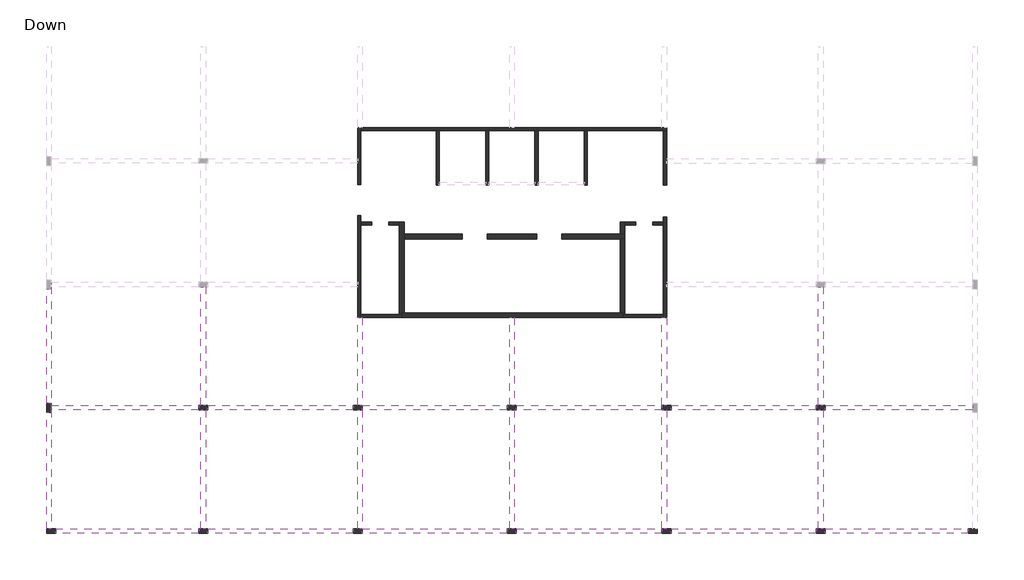
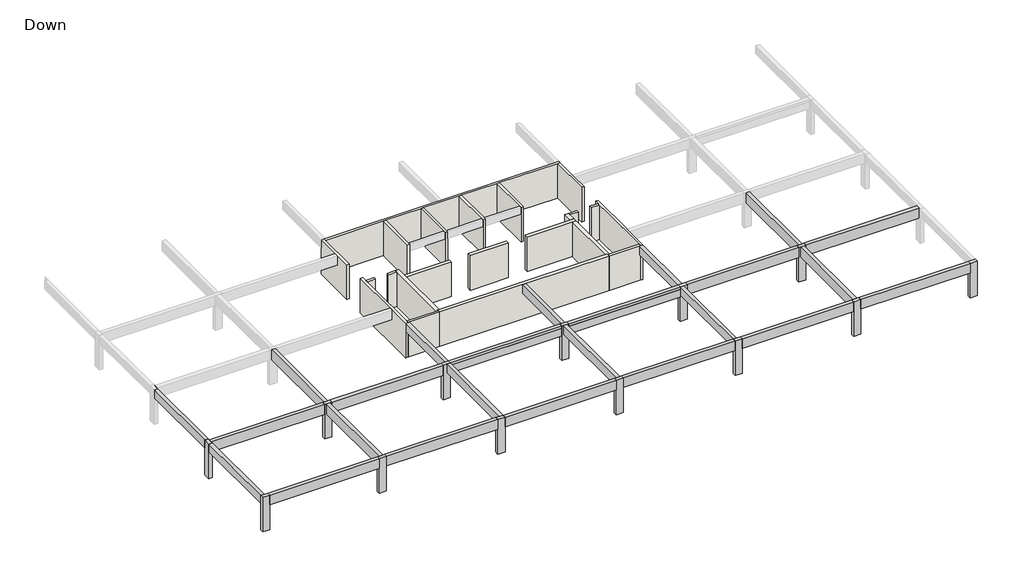
# One storey, part 1 of 2: 24 beams, 22 walls, 13 columns.
"""IFC4 building model written with IfcOpenShell, lengths in millimetres."""

import ifcopenshell
import ifcopenshell.guid

model = None  # the IFC model being written
_history = None  # IfcOwnerHistory: only IFC2X3 demands one
_inside = {}  # id of a spatial element -> (the spatial element, [elements in it])
_under = {}  # id of a project, library or spatial element -> (it, [spatial elements below it])
_declared = {}  # id of a project -> (the project, [libraries it declares])
_typed = {}  # id of a type object -> (the type object, [elements of that type])
_made_of = {}  # id of a material, layer set ... -> (it, [elements and type objects made of it])


def new_model(schema):
    """Start an empty IFC model of exactly this schema.

    Asked for "IFC4X3", IfcOpenShell would pick the latest addendum, in which some entities
    have other attributes; the version numbers below select the first issue.
    IFC2X3 requires an IfcOwnerHistory on every rooted entity: one is made here for all.
    """
    global model, _history
    if schema == "IFC4X3":
        model = ifcopenshell.file(schema_version=(4, 3, 0, 0))
    else:
        model = ifcopenshell.file(schema=schema)
    _inside.clear()
    _under.clear()
    _declared.clear()
    _typed.clear()
    _made_of.clear()
    _history = None
    if model.schema == "IFC2X3":
        org = make("IfcOrganization", Name="unknown")
        user = make(
            "IfcPersonAndOrganization",
            ThePerson=make("IfcPerson", FamilyName="unknown"),
            TheOrganization=org,
        )
        app = make(
            "IfcApplication",
            ApplicationDeveloper=org,
            Version="unknown",
            ApplicationFullName="unknown",
            ApplicationIdentifier="unknown",
        )
        _history = make(
            "IfcOwnerHistory",
            OwningUser=user,
            OwningApplication=app,
            ChangeAction="ADDED",
            CreationDate=0,
        )
    return model


def make(cls, **values):
    """One entity of the class cls with the attributes given. An attribute that is None is left unset."""
    return model.create_entity(
        cls, **{name: value for name, value in values.items() if value is not None}
    )


def rooted(cls, **values):
    """An entity with a GlobalId (a new one), such as an element, a storey or a relation."""
    return make(cls, GlobalId=ifcopenshell.guid.new(), OwnerHistory=_history, **values)


def si_unit(unit_type, name, prefix=None):
    """IfcSIUnit, for example si_unit("LENGTHUNIT", "METRE", prefix="MILLI")."""
    return make("IfcSIUnit", UnitType=unit_type, Prefix=prefix, Name=name)


def assignment(units):
    """IfcUnitAssignment: the units of a project."""
    return None if units is None else make("IfcUnitAssignment", Units=units)


def point(xyz):
    """IfcCartesianPoint."""
    return None if xyz is None else make("IfcCartesianPoint", Coordinates=xyz)


def direction(xyz):
    """IfcDirection."""
    return None if xyz is None else make("IfcDirection", DirectionRatios=xyz)


def frame(location, z_axis=None, x_axis=None):
    """IfcAxis2Placement3D, a coordinate frame: its origin and axes. An axis left out is left unset."""
    return make(
        "IfcAxis2Placement3D",
        Location=point(location),
        Axis=direction(z_axis),
        RefDirection=direction(x_axis),
    )


def origin():
    """The frame at (0, 0, 0) with its axes left unset."""
    return frame((0.0, 0.0, 0.0))


def origin_with_axes():
    """The frame at (0, 0, 0) with the z axis (0, 0, 1) and the x axis (1, 0, 0) written out."""
    return frame((0.0, 0.0, 0.0), z_axis=(0.0, 0.0, 1.0), x_axis=(1.0, 0.0, 0.0))


def place(relative_to, where):
    """IfcLocalPlacement: puts the frame where relative to a parent placement (None: the world)."""
    return make(
        "IfcLocalPlacement", PlacementRelTo=relative_to, RelativePlacement=where
    )


def context(
    kind, dimensions, precision=None, world=None, true_north=None, identifier=None
):
    """IfcGeometricRepresentationContext, for example the 3D "Model" context."""
    return make(
        "IfcGeometricRepresentationContext",
        ContextIdentifier=identifier,
        ContextType=kind,
        CoordinateSpaceDimension=dimensions,
        Precision=precision,
        WorldCoordinateSystem=world,
        TrueNorth=true_north,
    )


def project(units=None, contexts=None):
    """IfcProject with its units and contexts."""
    return rooted(
        "IfcProject",
        Name="project",
        RepresentationContexts=contexts,
        UnitsInContext=assignment(units),
    )


def spatial(cls, under=None, at=None, **own):
    """A site, building, storey or space (cls), placed at a placement, below another one or the project."""
    s = rooted(cls, ObjectPlacement=at, **own)
    if under is not None:
        _under.setdefault(under.id(), (under, []))[1].append(s)
    return s


def polyline(points):
    """IfcPolyline through the points."""
    return make("IfcPolyline", Points=[point(p) for p in points])


def outline(outer, holes=None, kind="AREA"):
    """IfcArbitraryClosedProfileDef: a profile drawn as a closed curve; with holes, ...WithVoids."""
    if holes is None:
        return make("IfcArbitraryClosedProfileDef", ProfileType=kind, OuterCurve=outer)
    return make(
        "IfcArbitraryProfileDefWithVoids",
        ProfileType=kind,
        OuterCurve=outer,
        InnerCurves=holes,
    )


def extrude(swept, where, along, depth):
    """IfcExtrudedAreaSolid: the profile swept, set in the frame where, extruded along a direction by depth."""
    return make(
        "IfcExtrudedAreaSolid",
        SweptArea=swept,
        Position=where,
        ExtrudedDirection=direction(along),
        Depth=depth,
    )


def faces_of(points, faces, orient=None, outer=None):
    """IfcFace entities. A face is a list of loops; a loop is a list of indices into points, from 0.

    orient and outer hold one flag for each loop. By default every Orientation is true, the
    first loop of a face is its IfcFaceOuterBound and the others are IfcFaceBound.
    """
    made = []
    for i, loops in enumerate(faces):
        bounds = []
        for j, loop in enumerate(loops):
            is_outer = j == 0 if outer is None else outer[i][j]
            bounds.append(
                make(
                    "IfcFaceOuterBound" if is_outer else "IfcFaceBound",
                    Bound=make("IfcPolyLoop", Polygon=[points[k] for k in loop]),
                    Orientation=True if orient is None else orient[i][j],
                )
            )
        made.append(make("IfcFace", Bounds=bounds))
    return made


def faceted_brep(points, faces, orient=None, outer=None, voids=None):
    """IfcFacetedBrep: a solid bounded by flat faces; with voids (closed shells), ...WithVoids."""
    shared = [point(p) for p in points]
    hull = make("IfcClosedShell", CfsFaces=faces_of(shared, faces, orient, outer))
    if voids is None:
        return make("IfcFacetedBrep", Outer=hull)
    return make(
        "IfcFacetedBrepWithVoids",
        Outer=hull,
        Voids=[
            make(cls, CfsFaces=faces_of(shared, fs, o, b)) for cls, fs, o, b in voids
        ],
    )


def shape(context_of_items, identifier, shape_type, items):
    """IfcShapeRepresentation: the items that make up one representation, for example the "Body"."""
    return make(
        "IfcShapeRepresentation",
        ContextOfItems=context_of_items,
        RepresentationIdentifier=identifier,
        RepresentationType=shape_type,
        Items=items,
    )


def made_of(thing, what):
    """Note that an element or type object is made of a material, layer set ...; save() writes the relation."""
    if what is not None:
        _made_of.setdefault(what.id(), (what, []))[1].append(thing)
    return thing


def element(
    cls,
    number,
    at=None,
    inside=None,
    cuts=None,
    type_object=None,
    material=None,
    context=None,
    identifier="Body",
    shape_type=None,
    held_by="IfcProductDefinitionShape",
    body=None,
    shapes=None,
    **own,
):
    """One element of the class cls, such as IfcWall. Its Tag is "e" and its number.

    at: its placement. inside: the storey or other place that contains it. cuts: it is an
    opening in that element (IfcRelVoidsElement). A single representation is given by context,
    identifier, shape_type and body (its items); several are given by shapes. held_by: the class
    of the entity that holds the representations. save() writes the other relations.
    """
    e = rooted(cls, Tag="e%d" % number, ObjectPlacement=at, **own)
    if body is not None:
        shapes = [shape(context, identifier, shape_type, body)]
    if shapes is not None:
        e.Representation = make(held_by, Representations=shapes)
    if inside is not None:
        _inside.setdefault(inside.id(), (inside, []))[1].append(e)
    if cuts is not None:
        rooted(
            "IfcRelVoidsElement", RelatingBuildingElement=cuts, RelatedOpeningElement=e
        )
    if type_object is not None:
        _typed.setdefault(type_object.id(), (type_object, []))[1].append(e)
    return made_of(e, material)


def aggregate(whole, parts):
    """IfcRelAggregates: a whole, such as a stair, and the parts it consists of."""
    return rooted("IfcRelAggregates", RelatingObject=whole, RelatedObjects=parts)


def save(model, path):
    """Write the relations noted so far, then the file.

    IfcRelAggregates (storeys below a building ...), IfcRelContainedInSpatialStructure (elements
    in a storey), IfcRelDefinesByType, IfcRelAssociatesMaterial and IfcRelDeclares: one each for
    every whole, place, type object, material and project.
    """
    for whole, parts in _under.values():
        aggregate(whole, parts)
    for where, things in _inside.values():
        rooted(
            "IfcRelContainedInSpatialStructure",
            RelatedElements=things,
            RelatingStructure=where,
        )
    for kind, things in _typed.values():
        rooted("IfcRelDefinesByType", RelatedObjects=things, RelatingType=kind)
    for what, things in _made_of.values():
        rooted("IfcRelAssociatesMaterial", RelatedObjects=things, RelatingMaterial=what)
    for by, libraries in _declared.values():
        rooted("IfcRelDeclares", RelatingContext=by, RelatedDefinitions=libraries)
    model.write(path)


model = new_model("IFC4")

# Units and contexts
model_context = context("Model", 3, world=origin())
ifc_project = project(units=[si_unit("LENGTHUNIT", "METRE", prefix="MILLI")], contexts=[model_context])

# Site, building, storey
site = spatial("IfcSite", under=ifc_project)
building = spatial("IfcBuilding", under=site)
storey = spatial("IfcBuildingStorey", under=building, Name="Down", Elevation=0.0)

# Beams
placement = place(None, origin())
element("IfcBeam", 1, ObjectType="Concrete Rectengular Beam : 30/70", at=placement, inside=storey, context=model_context, shape_type="Brep", body=[
    faceted_brep([(-26599.1167382, -14918.7716477, 3080.0), (-26299.1167382, -14918.7716477, 3080.0), (-26299.1167382, -7220.4648963, 3080.0), (-26299.1167382, -6920.4648963, 3080.0), (-26299.591421, -6920.4648963, 3080.0), (-26299.591421, -7370.4648963, 3080.0), (-26599.1167382, -7370.4648963, 3080.0), (-26299.1167382, -14918.7716477, 2860.0), (-26299.1167382, -14918.7716477, 2380.0), (-26299.1167382, -7220.4648963, 2380.0), (-26299.1167382, -6920.4648963, 2380.0), (-26599.1167382, -14918.7716477, 2380.0), (-26599.1167382, -7370.4648963, 2380.0), (-26299.591421, -7370.4648963, 2380.0), (-26299.591421, -7220.4648963, 2380.0), (-26299.591421, -6920.4648963, 2380.0)], [[[0, 1, 2, 3, 4, 5, 6]], [[1, 7, 8, 9, 10, 3, 2]], [[8, 11, 12, 13, 14, 15, 10, 9]], [[11, 0, 6, 12]], [[1, 0, 11, 8, 7]], [[13, 5, 4, 15, 14]], [[5, 13, 12, 6]], [[3, 10, 15, 4]]]),
])
element("IfcBeam", 2, ObjectType="Concrete Rectengular Beam : 30/70", at=placement, inside=storey, context=model_context, shape_type="Brep", body=[
    faceted_brep([(-26599.1167382, -6770.4648963, 3080.0), (-26299.591421, -6770.4648963, 3080.0), (-26299.591421, -6920.4648963, 3080.0), (-26299.1167382, -6920.4648963, 3080.0), (-26299.1167382, 774.102585, 3080.0), (-26299.1167382, 1074.102585, 3080.0), (-26299.591421, 1074.102585, 3080.0), (-26299.591421, 624.102585, 3080.0), (-26599.1167382, 624.102585, 3080.0), (-26299.1167382, 1074.102585, 2380.0), (-26299.1167382, -6920.4648963, 2860.0), (-26299.1167382, -6920.4648963, 2380.0), (-26299.1167382, 774.102585, 2380.0), (-26299.591421, -6770.4648963, 2380.0), (-26599.1167382, -6770.4648963, 2380.0), (-26599.1167382, 624.102585, 2380.0), (-26299.591421, 624.102585, 2380.0), (-26299.591421, 774.102585, 2380.0), (-26299.591421, 1074.102585, 2380.0), (-26299.591421, -6920.4648963, 2380.0)], [[[0, 1, 2, 3, 4, 5, 6, 7, 8]], [[9, 5, 4, 3, 10, 11, 12]], [[13, 14, 15, 16, 17, 18, 9, 12, 11, 19]], [[14, 0, 8, 15]], [[13, 1, 0, 14]], [[1, 13, 19, 2]], [[16, 7, 6, 18, 17]], [[7, 16, 15, 8]], [[5, 9, 18, 6]], [[11, 10, 3, 2, 19]]]),
])
element("IfcBeam", 3, ObjectType="Concrete Rectengular Beam : 30/75", at=placement, inside=storey, context=model_context, shape_type="Brep", body=[
    faceted_brep([(-6147.328783, -7220.4648963, 3080.0), (-6447.328783, -7220.4648963, 3080.0), (-6447.328783, -14918.7716477, 3080.0), (-6147.328783, -14918.7716477, 3080.0), (-6147.328783, -7220.4648963, 2330.0), (-6147.328783, -14918.7716477, 2330.0), (-6447.328783, -7220.4648963, 2330.0), (-6447.328783, -14918.7716477, 2330.0), (-6447.328783, -7220.4648963, 2860.0), (-6447.328783, -14918.7716477, 2860.0)], [[[0, 1, 2, 3]], [[4, 0, 3, 5]], [[6, 4, 5, 7]], [[1, 8, 6, 7, 9, 2]], [[1, 0, 4, 6, 8]], [[3, 2, 9, 7, 5]]]),
])
element("IfcBeam", 4, ObjectType="Concrete Rectengular Beam : 30/75", at=placement, inside=storey, context=model_context, shape_type="Brep", body=[
    faceted_brep([(-6447.328783, -6920.4648963, 3080.0), (-6147.328783, -6920.4648963, 3080.0), (-6147.328783, -1210.4648963, 3080.0), (-6247.328783, -1210.4648963, 3080.0), (-6447.328783, -1210.4648963, 3080.0), (-6147.328783, -6920.4648963, 2860.0), (-6147.328783, -6920.4648963, 2330.0), (-6147.328783, -1210.4648963, 2330.0), (-6147.328783, -1210.4648963, 2860.0), (-6447.328783, -6920.4648963, 2330.0), (-6447.328783, -1210.4648963, 2330.0), (-6447.328783, -6920.4648963, 2860.0)], [[[0, 1, 2, 3, 4]], [[1, 5, 6, 7, 8, 2]], [[6, 9, 10, 7]], [[9, 11, 0, 4, 10]], [[1, 0, 11, 9, 6, 5]], [[2, 8, 7, 10, 4, 3]]]),
])
element("IfcBeam", 5, ObjectType="Concrete Rectengular Beam : 30/75", at=placement, inside=storey, context=model_context, shape_type="Brep", body=[
    faceted_brep([(3389.2018335, -6920.4648963, 3080.0), (3689.2018335, -6920.4648963, 3080.0), (3689.2018335, -1210.4648963, 3080.0), (3389.2018335, -1210.4648963, 3080.0), (3689.2018335, -6920.4648963, 2860.0), (3689.2018335, -6920.4648963, 2330.0), (3689.2018335, -1210.4648963, 2330.0), (3689.2018335, -1210.4648963, 2860.0), (3389.2018335, -6920.4648963, 2330.0), (3389.2018335, -1210.4648963, 2330.0), (3389.2018335, -6920.4648963, 2860.0), (3389.2018335, -1210.4648963, 2860.0)], [[[0, 1, 2, 3]], [[1, 4, 5, 6, 7, 2]], [[5, 8, 9, 6]], [[8, 10, 0, 3, 11, 9]], [[1, 0, 10, 8, 5, 4]], [[3, 2, 7, 6, 9, 11]]]),
])
element("IfcBeam", 6, ObjectType="Concrete Rectengular Beam : 30/75", at=placement, inside=storey, context=model_context, shape_type="Brep", body=[
    faceted_brep([(3389.2018335, -14918.7716477, 3080.0), (3689.2018335, -14918.7716477, 3080.0), (3689.2018335, -7220.4648963, 3080.0), (3389.2018335, -7220.4648963, 3080.0), (3389.2018335, -14918.7716477, 2330.0), (3389.2018335, -14918.7716477, 2860.0), (3389.2018335, -7220.4648963, 2860.0), (3389.2018335, -7220.4648963, 2330.0), (3689.2018335, -14918.7716477, 2330.0), (3689.2018335, -7220.4648963, 2330.0), (3689.2018335, -14918.7716477, 2860.0), (3689.2018335, -7220.4648963, 2860.0)], [[[0, 1, 2, 3]], [[4, 5, 0, 3, 6, 7]], [[8, 4, 7, 9]], [[1, 10, 8, 9, 11, 2]], [[1, 0, 5, 4, 8, 10]], [[3, 2, 11, 9, 7, 6]]]),
])
element("IfcBeam", 7, ObjectType="Concrete Rectengular Beam : 30/75", at=placement, inside=storey, context=model_context, shape_type="SweptSolid", body=[
    extrude(outline(polyline([(2330.0, 13257.9839294), (2330.0, 13557.9839294), (2860.0, 13557.9839294), (2860.0, 13525.73245), (3080.0, 13525.73245), (3080.0, 13257.9839294), (2330.0, 13257.9839294)])), frame((0.0, -14918.7716477, 0.0), z_axis=(0.0, 1.0, 0.0), x_axis=(0.0, 0.0, 1.0)), (0.0, 0.0, 1.0), 7698.3067514),
])
element("IfcBeam", 8, ObjectType="Concrete Rectengular Beam : 30/75", at=placement, inside=storey, context=model_context, shape_type="Brep", body=[
    faceted_brep([(13257.9839294, -6920.4648963, 3080.0), (13557.9839294, -6920.4648963, 3080.0), (13557.9839294, -1210.4648963, 3080.0), (13357.9839294, -1210.4648963, 3080.0), (13257.9839294, -1210.4648963, 3080.0), (13557.9839294, -6920.4648963, 2860.0), (13557.9839294, -6920.4648963, 2330.0), (13557.9839294, -1210.4648963, 2330.0), (13257.9839294, -6920.4648963, 2330.0), (13257.9839294, -1210.4648963, 2330.0), (13257.9839294, -6920.4648963, 2860.0), (13257.9839294, -1210.4648963, 2860.0)], [[[0, 1, 2, 3, 4]], [[1, 5, 6, 7, 2]], [[6, 8, 9, 7]], [[8, 10, 0, 4, 11, 9]], [[1, 0, 10, 8, 6, 5]], [[2, 7, 9, 11, 4, 3]]]),
])
element("IfcBeam", 9, ObjectType="Concrete Rectengular Beam : 30/85", at=placement, inside=storey, context=model_context, shape_type="SweptSolid", body=[
    extrude(outline(polyline([(33098.6447783, -14918.7716477), (33098.6447783, -15218.7716477), (23850.3644839, -15218.7716477), (23850.3644839, -14918.7716477), (33098.6447783, -14918.7716477)])), frame((0.0, 0.0, 2230.0), z_axis=(0.0, 0.0, 1.0), x_axis=(1.0, 0.0, 0.0)), (0.0, 0.0, 1.0), 850.0),
])
element("IfcBeam", 10, ObjectType="Concrete Rectengular Beam : 30/85", at=placement, inside=storey, context=model_context, shape_type="SweptSolid", body=[
    extrude(outline(polyline([(23250.3644839, -14918.7716477), (23250.3644839, -15218.7716477), (13857.9839294, -15218.7716477), (13857.9839294, -14918.7716477), (23250.3644839, -14918.7716477)])), frame((0.0, 0.0, 2230.0), z_axis=(0.0, 0.0, 1.0), x_axis=(1.0, 0.0, 0.0)), (0.0, 0.0, 1.0), 850.0),
])
element("IfcBeam", 11, ObjectType="Concrete Rectengular Beam : 30/85", at=placement, inside=storey, context=model_context, shape_type="SweptSolid", body=[
    extrude(outline(polyline([(-14918.7716477, 2230.0), (-15218.7716477, 2230.0), (-15218.7716477, 3080.0), (-14922.522162, 3080.0), (-14922.522162, 2860.0), (-14918.7716477, 2860.0), (-14918.7716477, 2230.0)])), frame((3839.2018335, 0.0, 0.0), z_axis=(1.0, 0.0, 0.0), x_axis=(0.0, 1.0, 0.0)), (0.0, 0.0, 1.0), 9418.7820959),
])
element("IfcBeam", 12, ObjectType="Concrete Rectengular Beam : 30/85", at=placement, inside=storey, context=model_context, shape_type="SweptSolid", body=[
    extrude(outline(polyline([(-14918.7716477, 2230.0), (-15218.7716477, 2230.0), (-15218.7716477, 3080.0), (-14922.522162, 3080.0), (-14922.522162, 2860.0), (-14918.7716477, 2860.0), (-14918.7716477, 2230.0)])), frame((-6147.328783, 0.0, 0.0), z_axis=(1.0, 0.0, 0.0), x_axis=(0.0, 1.0, 0.0)), (0.0, 0.0, 1.0), 9386.5306165),
])
element("IfcBeam", 13, ObjectType="Concrete Rectengular Beam : 30/85", at=placement, inside=storey, context=model_context, shape_type="SweptSolid", body=[
    extrude(outline(polyline([(-16150.7819865, -15218.7716477), (-16150.7819865, -14918.7716477), (-6747.328783, -14918.7716477), (-6747.328783, -15218.7716477), (-16150.7819865, -15218.7716477)])), frame((0.0, 0.0, 2230.0), z_axis=(0.0, 0.0, 1.0), x_axis=(1.0, 0.0, 0.0)), (0.0, 0.0, 1.0), 850.0),
])
element("IfcBeam", 14, ObjectType="Concrete Rectengular Beam : 30/85", at=placement, inside=storey, context=model_context, shape_type="SweptSolid", body=[
    extrude(outline(polyline([(-25999.1167382, -15218.7716477), (-25999.1167382, -14918.7716477), (-16750.7819865, -14918.7716477), (-16750.7819865, -15218.7716477), (-25999.1167382, -15218.7716477)])), frame((0.0, 0.0, 2230.0), z_axis=(0.0, 0.0, 1.0), x_axis=(1.0, 0.0, 0.0)), (0.0, 0.0, 1.0), 850.0),
])
element("IfcBeam", 15, ObjectType="Concrete Rectengular Beam : 30/90", at=placement, inside=storey, context=model_context, shape_type="Brep", body=[
    faceted_brep([(-16750.7819865, -7220.4648963, 3080.0), (-16750.7819865, -6920.4648963, 3080.0), (-26299.1167382, -6920.4648963, 3080.0), (-26299.1167382, -7220.4648963, 3080.0), (-16750.7819865, -7220.4648963, 2180.0), (-26299.1167382, -7220.4648963, 2860.0), (-26299.1167382, -7220.4648963, 2380.0), (-26299.591421, -7220.4648963, 2380.0), (-26299.591421, -7220.4648963, 2180.0), (-16750.7819865, -6920.4648963, 2180.0), (-26299.591421, -6920.4648963, 2180.0), (-26299.591421, -6920.4648963, 2380.0), (-26299.1167382, -6920.4648963, 2380.0), (-26299.1167382, -6920.4648963, 2860.0)], [[[0, 1, 2, 3]], [[4, 0, 3, 5, 6, 7, 8]], [[9, 4, 8, 10]], [[1, 9, 10, 11, 12, 13, 2]], [[1, 0, 4, 9]], [[10, 8, 7, 11]], [[12, 6, 5, 3, 2, 13]], [[6, 12, 11, 7]]]),
])
element("IfcBeam", 16, ObjectType="Concrete Rectengular Beam : 30/90", at=placement, inside=storey, context=model_context, shape_type="SweptSolid", body=[
    extrude(outline(polyline([(-16150.7819865, -7220.4648963), (-16150.7819865, -6920.4648963), (-6747.328783, -6920.4648963), (-6747.328783, -7220.4648963), (-16150.7819865, -7220.4648963)])), frame((0.0, 0.0, 2180.0), z_axis=(0.0, 0.0, 1.0), x_axis=(1.0, 0.0, 0.0)), (0.0, 0.0, 1.0), 900.0),
])
element("IfcBeam", 17, ObjectType="Concrete Rectengular Beam : 30/90", at=placement, inside=storey, context=model_context, shape_type="Brep", body=[
    faceted_brep([(3239.2018335, -6920.4648963, 3080.0), (-6147.328783, -6920.4648963, 3080.0), (-6147.328783, -7220.13739, 3080.0), (3239.2018335, -7220.13739, 3080.0), (-6147.328783, -7220.4648963, 2180.0), (3239.2018335, -7220.4648963, 2180.0), (3239.2018335, -7220.4648963, 2860.0), (-6147.328783, -7220.4648963, 2860.0), (3239.2018335, -6920.4648963, 2180.0), (-6147.328783, -6920.4648963, 2180.0), (-6147.328783, -6920.4648963, 2860.0), (3239.2018335, -7220.13739, 2860.0), (-6147.328783, -7220.13739, 2860.0)], [[[0, 1, 2, 3]], [[4, 5, 6, 7]], [[8, 5, 4, 9]], [[0, 8, 9, 10, 1]], [[5, 8, 0, 3, 11, 6]], [[9, 4, 7, 12, 2, 1, 10]], [[11, 12, 7, 6]], [[12, 11, 3, 2]]]),
])
element("IfcBeam", 18, ObjectType="Concrete Rectengular Beam : 30/90", at=placement, inside=storey, context=model_context, shape_type="Brep", body=[
    faceted_brep([(13257.9839294, -6920.4648963, 3080.0), (3839.2018335, -6920.4648963, 3080.0), (3839.2018335, -7220.13739, 3080.0), (13257.9839294, -7220.13739, 3080.0), (3839.2018335, -7220.4648963, 2180.0), (13257.9839294, -7220.4648963, 2180.0), (13257.9839294, -7220.4648963, 2860.0), (3839.2018335, -7220.4648963, 2860.0), (3839.2018335, -6920.4648963, 2180.0), (13257.9839294, -6920.4648963, 2180.0), (13257.9839294, -6920.4648963, 2860.0), (3839.2018335, -7220.13739, 2860.0), (13257.9839294, -7220.13739, 2860.0)], [[[0, 1, 2, 3]], [[4, 5, 6, 7]], [[4, 8, 9, 5]], [[8, 1, 0, 10, 9]], [[8, 4, 7, 11, 2, 1]], [[5, 9, 10, 0, 3, 12, 6]], [[12, 11, 7, 6]], [[11, 12, 3, 2]]]),
])
element("IfcBeam", 19, ObjectType="Concrete Rectengular Beam : 30/90", at=placement, inside=storey, context=model_context, shape_type="SweptSolid", body=[
    extrude(outline(polyline([(23250.3644839, -6920.4648963), (23250.3644839, -7220.4648963), (13857.9839294, -7220.4648963), (13857.9839294, -6920.4648963), (23250.3644839, -6920.4648963)])), frame((0.0, 0.0, 2180.0), z_axis=(0.0, 0.0, 1.0), x_axis=(1.0, 0.0, 0.0)), (0.0, 0.0, 1.0), 900.0),
])
element("IfcBeam", 20, ObjectType="Concrete Rectengular Beam : 30/90", at=placement, inside=storey, context=model_context, shape_type="Brep", body=[
    faceted_brep([(33398.6447783, -7220.4648963, 3080.0), (33398.6447783, -6920.4648963, 3080.0), (23850.3644839, -6920.4648963, 3080.0), (23850.3644839, -7220.4648963, 3080.0), (33398.6447783, -7220.4648963, 2180.0), (33398.6447783, -7220.4648963, 2860.0), (23850.3644839, -7220.4648963, 2180.0), (33398.6447783, -6920.4648963, 2180.0), (23850.3644839, -6920.4648963, 2180.0), (33398.6447783, -6920.4648963, 2860.0)], [[[0, 1, 2, 3]], [[4, 5, 0, 3, 6]], [[7, 4, 6, 8]], [[1, 9, 7, 8, 2]], [[1, 0, 5, 4, 7, 9]], [[3, 2, 8, 6]]]),
])
element("IfcBeam", 21, ObjectType="Concrete Rectengular Beam : 30/90", at=placement, inside=storey, context=model_context, shape_type="Brep", body=[
    faceted_brep([(-16600.7819865, -6920.4648963, 3080.0), (-16300.7819865, -6920.4648963, 3080.0), (-16300.7819865, 774.102585, 3080.0), (-16600.7819865, 774.102585, 3080.0), (-16600.7819865, -6920.4648963, 2180.0), (-16600.7819865, -6920.4648963, 2860.0), (-16600.7819865, 774.102585, 2860.0), (-16600.7819865, 774.102585, 2180.0), (-16300.7819865, -6920.4648963, 2180.0), (-16300.7819865, 774.102585, 2180.0), (-16300.7819865, -6920.4648963, 2860.0), (-16300.7819865, 774.102585, 2860.0)], [[[0, 1, 2, 3]], [[4, 5, 0, 3, 6, 7]], [[8, 4, 7, 9]], [[1, 10, 8, 9, 11, 2]], [[0, 5, 4, 8, 10, 1]], [[2, 11, 9, 7, 6, 3]]]),
])
element("IfcBeam", 22, ObjectType="Concrete Rectengular Beam : 30/90", at=placement, inside=storey, context=model_context, shape_type="Brep", body=[
    faceted_brep([(-16300.7819865, -7220.4648963, 3080.0), (-16600.7819865, -7220.4648963, 3080.0), (-16600.7819865, -14918.7716477, 3080.0), (-16300.7819865, -14918.7716477, 3080.0), (-16600.7819865, -7220.4648963, 2860.0), (-16600.7819865, -7220.4648963, 2180.0), (-16600.7819865, -14918.7716477, 2180.0), (-16600.7819865, -14918.7716477, 2860.0), (-16300.7819865, -7220.4648963, 2180.0), (-16300.7819865, -14918.7716477, 2180.0), (-16300.7819865, -7220.4648963, 2860.0), (-16300.7819865, -14918.7716477, 2860.0)], [[[0, 1, 2, 3]], [[1, 4, 5, 6, 7, 2]], [[5, 8, 9, 6]], [[8, 10, 0, 3, 11, 9]], [[5, 4, 1, 0, 10, 8]], [[3, 2, 7, 6, 9, 11]]]),
])
element("IfcBeam", 23, ObjectType="Concrete Rectengular Beam : 30/90", at=placement, inside=storey, context=model_context, shape_type="Brep", body=[
    faceted_brep([(23400.3644839, -6920.4648963, 3080.0), (23700.3644839, -6920.4648963, 3080.0), (23700.3644839, 774.102585, 3080.0), (23400.3644839, 774.102585, 3080.0), (23400.3644839, -6920.4648963, 2180.0), (23400.3644839, -6920.4648963, 2860.0), (23400.3644839, 774.102585, 2860.0), (23400.3644839, 774.102585, 2180.0), (23700.3644839, -6920.4648963, 2180.0), (23700.3644839, 774.102585, 2180.0), (23700.3644839, -6920.4648963, 2860.0), (23700.3644839, 774.102585, 2860.0)], [[[0, 1, 2, 3]], [[4, 5, 0, 3, 6, 7]], [[8, 4, 7, 9]], [[1, 10, 8, 9, 11, 2]], [[0, 5, 4, 8, 10, 1]], [[9, 7, 6, 3, 2, 11]]]),
])
element("IfcBeam", 24, ObjectType="Concrete Rectengular Beam : 30/90", at=placement, inside=storey, context=model_context, shape_type="Brep", body=[
    faceted_brep([(23700.3644839, -7220.4648963, 3080.0), (23400.3644839, -7220.4648963, 3080.0), (23400.3644839, -14918.7716477, 3080.0), (23700.3644839, -14918.7716477, 3080.0), (23400.3644839, -7220.4648963, 2860.0), (23400.3644839, -7220.4648963, 2180.0), (23400.3644839, -14918.7716477, 2180.0), (23400.3644839, -14918.7716477, 2860.0), (23700.3644839, -7220.4648963, 2180.0), (23700.3644839, -14918.7716477, 2180.0), (23700.3644839, -7220.4648963, 2860.0), (23700.3644839, -14918.7716477, 2860.0)], [[[0, 1, 2, 3]], [[1, 4, 5, 6, 7, 2]], [[5, 8, 9, 6]], [[8, 10, 0, 3, 11, 9]], [[5, 4, 1, 0, 10, 8]], [[3, 2, 7, 6, 9, 11]]]),
])

# Columns
element("IfcColumn", 25, ObjectType="Concrete Rectengular Column : 30/60", at=placement, inside=storey, context=model_context, shape_type="Brep", body=[
    faceted_brep([(33098.6447783, -14918.7716477, 0.0), (33698.6447783, -14918.7716477, 0.0), (33698.6447783, -15218.7716477, 0.0), (33098.6447783, -15218.7716477, 0.0), (33098.6447783, -14918.7716477, 3080.0), (33398.6447783, -14918.7716477, 3080.0), (33698.6447783, -14918.7716477, 3080.0), (33698.6447783, -15218.7716477, 3080.0), (33098.6447783, -15218.7716477, 3080.0)], [[[0, 1, 2, 3]], [[4, 5, 6, 1, 0]], [[6, 7, 2, 1]], [[7, 8, 3, 2]], [[8, 4, 0, 3]], [[4, 8, 7, 6, 5]]]),
])
element("IfcColumn", 26, ObjectType="Concrete Rectengular Column : 30/60", at=placement, inside=storey, context=model_context, shape_type="Brep", body=[
    faceted_brep([(23250.3644839, -6920.4648963, 0.0), (23850.3644839, -6920.4648963, 0.0), (23850.3644839, -7220.4648963, 0.0), (23250.3644839, -7220.4648963, 0.0), (23250.3644839, -6920.4648963, 3080.0), (23400.3644839, -6920.4648963, 3080.0), (23700.3644839, -6920.4648963, 3080.0), (23850.3644839, -6920.4648963, 3080.0), (23850.3644839, -7220.4648963, 3080.0), (23700.3644839, -7220.4648963, 3080.0), (23400.3644839, -7220.4648963, 3080.0), (23250.3644839, -7220.4648963, 3080.0)], [[[0, 1, 2, 3]], [[4, 5, 6, 7, 1, 0]], [[7, 8, 2, 1]], [[8, 9, 10, 11, 3, 2]], [[11, 4, 0, 3]], [[4, 11, 10, 9, 8, 7, 6, 5]]]),
])
element("IfcColumn", 27, ObjectType="Concrete Rectengular Column : 30/60", at=placement, inside=storey, context=model_context, shape_type="Brep", body=[
    faceted_brep([(23250.3644839, -14918.7716477, 0.0), (23850.3644839, -14918.7716477, 0.0), (23850.3644839, -15218.7716477, 0.0), (23250.3644839, -15218.7716477, 0.0), (23250.3644839, -14918.7716477, 3080.0), (23400.3644839, -14918.7716477, 3080.0), (23700.3644839, -14918.7716477, 3080.0), (23850.3644839, -14918.7716477, 3080.0), (23850.3644839, -15218.7716477, 3080.0), (23250.3644839, -15218.7716477, 3080.0)], [[[0, 1, 2, 3]], [[4, 5, 6, 7, 1, 0]], [[7, 8, 2, 1]], [[8, 9, 3, 2]], [[9, 4, 0, 3]], [[4, 9, 8, 7, 6, 5]]]),
])
element("IfcColumn", 28, ObjectType="Concrete Rectengular Column : 30/60", at=placement, inside=storey, context=model_context, shape_type="Brep", body=[
    faceted_brep([(-26599.1167382, -14918.7716477, 0.0), (-25999.1167382, -14918.7716477, 0.0), (-25999.1167382, -15218.7716477, 0.0), (-26599.1167382, -15218.7716477, 0.0), (-26599.1167382, -14918.7716477, 3080.0), (-26299.1167382, -14918.7716477, 3080.0), (-25999.1167382, -14918.7716477, 3080.0), (-25999.1167382, -15218.7716477, 3080.0), (-26599.1167382, -15218.7716477, 3080.0)], [[[0, 1, 2, 3]], [[4, 5, 6, 1, 0]], [[6, 7, 2, 1]], [[7, 8, 3, 2]], [[8, 4, 0, 3]], [[4, 8, 7, 6, 5]]]),
])
element("IfcColumn", 29, ObjectType="Concrete Rectengular Column : 30/60", at=placement, inside=storey, context=model_context, shape_type="Brep", body=[
    faceted_brep([(-16750.7819865, -6920.4648963, 0.0), (-16150.7819865, -6920.4648963, 0.0), (-16150.7819865, -7220.4648963, 0.0), (-16750.7819865, -7220.4648963, 0.0), (-16750.7819865, -6920.4648963, 3080.0), (-16600.7819865, -6920.4648963, 3080.0), (-16300.7819865, -6920.4648963, 3080.0), (-16150.7819865, -6920.4648963, 3080.0), (-16150.7819865, -7220.4648963, 3080.0), (-16300.7819865, -7220.4648963, 3080.0), (-16600.7819865, -7220.4648963, 3080.0), (-16750.7819865, -7220.4648963, 3080.0)], [[[0, 1, 2, 3]], [[4, 5, 6, 7, 1, 0]], [[7, 8, 2, 1]], [[8, 9, 10, 11, 3, 2]], [[11, 4, 0, 3]], [[4, 11, 10, 9, 8, 7, 6, 5]]]),
])
element("IfcColumn", 30, ObjectType="Concrete Rectengular Column : 30/60", at=placement, inside=storey, context=model_context, shape_type="Brep", body=[
    faceted_brep([(-16750.7819865, -14918.7716477, 0.0), (-16150.7819865, -14918.7716477, 0.0), (-16150.7819865, -15218.7716477, 0.0), (-16750.7819865, -15218.7716477, 0.0), (-16750.7819865, -14918.7716477, 3080.0), (-16600.7819865, -14918.7716477, 3080.0), (-16300.7819865, -14918.7716477, 3080.0), (-16150.7819865, -14918.7716477, 3080.0), (-16150.7819865, -15218.7716477, 3080.0), (-16750.7819865, -15218.7716477, 3080.0)], [[[0, 1, 2, 3]], [[4, 5, 6, 7, 1, 0]], [[7, 8, 2, 1]], [[8, 9, 3, 2]], [[9, 4, 0, 3]], [[4, 9, 8, 7, 6, 5]]]),
])
element("IfcColumn", 31, ObjectType="Concrete Rectengular Column : 30/60", at=placement, inside=storey, context=model_context, shape_type="Brep", body=[
    faceted_brep([(3239.2018335, -14918.7716477, 0.0), (3839.2018335, -14918.7716477, 0.0), (3839.2018335, -15218.7716477, 0.0), (3239.2018335, -15218.7716477, 0.0), (3239.2018335, -14918.7716477, 3080.0), (3389.2018335, -14918.7716477, 3080.0), (3689.2018335, -14918.7716477, 3080.0), (3839.2018335, -14918.7716477, 3080.0), (3839.2018335, -14918.7716477, 2860.0), (3239.2018335, -14918.7716477, 2860.0), (3839.2018335, -14922.522162, 3080.0), (3839.2018335, -15218.7716477, 3080.0), (3239.2018335, -15218.7716477, 3080.0), (3239.2018335, -14922.522162, 3080.0)], [[[0, 1, 2, 3]], [[4, 5, 6, 7, 8, 1, 0, 9]], [[7, 10, 11, 2, 1, 8]], [[11, 12, 3, 2]], [[12, 13, 4, 9, 0, 3]], [[4, 13, 12, 11, 10, 7, 6, 5]]]),
])
element("IfcColumn", 32, ObjectType="Concrete Rectengular Column : 30/60", at=placement, inside=storey, context=model_context, shape_type="Brep", body=[
    faceted_brep([(3239.2018335, -6920.4648963, 0.0), (3839.2018335, -6920.4648963, 0.0), (3839.2018335, -7220.4648963, 0.0), (3239.2018335, -7220.4648963, 0.0), (3239.2018335, -6920.4648963, 3080.0), (3389.2018335, -6920.4648963, 3080.0), (3689.2018335, -6920.4648963, 3080.0), (3839.2018335, -6920.4648963, 3080.0), (3839.2018335, -7220.13739, 3080.0), (3839.2018335, -7220.4648963, 3080.0), (3839.2018335, -7220.4648963, 2860.0), (3689.2018335, -7220.4648963, 3080.0), (3389.2018335, -7220.4648963, 3080.0), (3239.2018335, -7220.4648963, 3080.0), (3239.2018335, -7220.4648963, 2860.0), (3239.2018335, -7220.13739, 3080.0)], [[[0, 1, 2, 3]], [[4, 5, 6, 7, 1, 0]], [[7, 8, 9, 10, 2, 1]], [[9, 11, 12, 13, 14, 3, 2, 10]], [[13, 15, 4, 0, 3, 14]], [[4, 15, 13, 12, 11, 9, 8, 7, 6, 5]]]),
])
element("IfcColumn", 33, ObjectType="Concrete Rectengular Column : 30/60", at=placement, inside=storey, context=model_context, shape_type="Brep", body=[
    faceted_brep([(-6747.328783, -6920.4648963, 0.0), (-6147.328783, -6920.4648963, 0.0), (-6147.328783, -7220.4648963, 0.0), (-6747.328783, -7220.4648963, 0.0), (-6747.328783, -6920.4648963, 3080.0), (-6447.328783, -6920.4648963, 3080.0), (-6147.328783, -6920.4648963, 3080.0), (-6147.328783, -7220.13739, 3080.0), (-6147.328783, -7220.4648963, 3080.0), (-6447.328783, -7220.4648963, 3080.0), (-6747.328783, -7220.4648963, 3080.0)], [[[0, 1, 2, 3]], [[4, 5, 6, 1, 0]], [[6, 7, 8, 2, 1]], [[8, 9, 10, 3, 2]], [[10, 4, 0, 3]], [[4, 10, 9, 8, 7, 6, 5]]]),
])
element("IfcColumn", 34, ObjectType="Concrete Rectengular Column : 30/60", at=placement, inside=storey, context=model_context, shape_type="Brep", body=[
    faceted_brep([(-6747.328783, -14918.7716477, 0.0), (-6147.328783, -14918.7716477, 0.0), (-6147.328783, -15218.7716477, 0.0), (-6747.328783, -15218.7716477, 0.0), (-6747.328783, -14918.7716477, 3080.0), (-6447.328783, -14918.7716477, 3080.0), (-6147.328783, -14918.7716477, 3080.0), (-6147.328783, -14922.522162, 3080.0), (-6147.328783, -15218.7716477, 3080.0), (-6747.328783, -15218.7716477, 3080.0)], [[[0, 1, 2, 3]], [[4, 5, 6, 1, 0]], [[6, 7, 8, 2, 1]], [[8, 9, 3, 2]], [[9, 4, 0, 3]], [[4, 9, 8, 7, 6, 5]]]),
])
element("IfcColumn", 35, ObjectType="Concrete Rectengular Column : 30/60", at=placement, inside=storey, context=model_context, shape_type="SweptSolid", body=[
    extrude(outline(polyline([(-26599.591421, -7370.4648963), (-26599.591421, -6770.4648963), (-26299.591421, -6770.4648963), (-26299.591421, -7370.4648963), (-26599.591421, -7370.4648963)])), origin_with_axes(), (0.0, 0.0, 1.0), 3080.0),
])
element("IfcColumn", 36, ObjectType="Concrete Rectengular Column : 30/60", at=placement, inside=storey, context=model_context, shape_type="Brep", body=[
    faceted_brep([(13257.9839294, -14918.7716477, 0.0), (13857.9839294, -14918.7716477, 0.0), (13857.9839294, -15218.7716477, 0.0), (13257.9839294, -15218.7716477, 0.0), (13257.9839294, -14918.7716477, 3080.0), (13525.73245, -14918.7716477, 3080.0), (13857.9839294, -14918.7716477, 3080.0), (13857.9839294, -15218.7716477, 3080.0), (13257.9839294, -15218.7716477, 3080.0), (13257.9839294, -14922.522162, 3080.0)], [[[0, 1, 2, 3]], [[4, 5, 6, 1, 0]], [[6, 7, 2, 1]], [[7, 8, 3, 2]], [[8, 9, 4, 0, 3]], [[4, 9, 8, 7, 6, 5]]]),
])
element("IfcColumn", 37, ObjectType="Concrete Rectengular Column : 30/60", at=placement, inside=storey, context=model_context, shape_type="Brep", body=[
    faceted_brep([(13257.9839294, -6920.4648963, 0.0), (13857.9839294, -6920.4648963, 0.0), (13857.9839294, -7220.4648963, 0.0), (13257.9839294, -7220.4648963, 0.0), (13257.9839294, -6920.4648963, 3080.0), (13557.9839294, -6920.4648963, 3080.0), (13857.9839294, -6920.4648963, 3080.0), (13857.9839294, -7220.4648963, 3080.0), (13525.73245, -7220.4648963, 3080.0), (13257.9839294, -7220.4648963, 3080.0), (13257.9839294, -7220.13739, 3080.0)], [[[0, 1, 2, 3]], [[4, 5, 6, 1, 0]], [[6, 7, 2, 1]], [[7, 8, 9, 3, 2]], [[9, 10, 4, 0, 3]], [[4, 10, 9, 8, 7, 6, 5]]]),
])

# Walls
element("IfcWall", 38, ObjectType="20", at=placement, inside=storey, context=model_context, shape_type="Brep", body=[
    faceted_brep([(-6247.328783, -1210.4648963, 0.0), (-6247.328783, -1010.4648963, 0.0), (-6247.328783, 4769.5351037, 0.0), (-6247.328783, 4969.5351037, 0.0), (-6247.328783, 5389.5351037, 0.0), (-6247.328783, 5389.5351037, 2860.0), (-6247.328783, 5389.5351037, 3080.0), (-6247.328783, 4969.5351037, 3080.0), (-6247.328783, 4769.5351037, 3080.0), (-6247.328783, 3781.3337247, 3080.0), (-6247.328783, -1010.4648963, 3080.0), (-6247.328783, -1210.4648963, 3080.0), (-6447.328783, -1210.4648963, 0.0), (-6447.328783, -1210.4648963, 2330.0), (-6447.328783, -1210.4648963, 3080.0), (-6447.328783, 774.102585, 3080.0), (-6447.328783, 1074.102585, 3080.0), (-6447.328783, 5389.5351037, 3080.0), (-6447.328783, 5389.5351037, 2860.0), (-6447.328783, 5389.5351037, 0.0), (-6442.328783, 5389.5351037, 3080.0)], [[[0, 1, 2, 3, 4, 5, 6, 7, 8, 9, 10, 11]], [[12, 13, 14, 15, 16, 17, 18, 19]], [[4, 3, 2, 1, 0, 12, 19]], [[6, 5, 4, 19, 18, 17, 20]], [[11, 10, 9, 8, 7, 6, 20, 17, 16, 15, 14]], [[0, 11, 14, 13, 12]]]),
])
element("IfcWall", 39, ObjectType="20", at=placement, inside=storey, context=model_context, shape_type="Brep", body=[
    faceted_brep([(-6247.328783, 7389.5351037, 0.0), (-6247.328783, 10889.5351037, 0.0), (-6247.328783, 11089.5351037, 0.0), (-6247.328783, 11089.5351037, 3080.0), (-6247.328783, 10889.5351037, 3080.0), (-6247.328783, 7389.5351037, 3080.0), (-6247.328783, 7389.5351037, 2860.0), (-6447.328783, 7389.5351037, 0.0), (-6447.328783, 7389.5351037, 2860.0), (-6447.328783, 7389.5351037, 3080.0), (-6447.328783, 8778.7943074, 3080.0), (-6447.328783, 9078.7943074, 3080.0), (-6447.328783, 11089.5351037, 3080.0), (-6447.328783, 11089.5351037, 2330.0), (-6447.328783, 11089.5351037, 0.0), (-6442.328783, 7389.5351037, 3080.0)], [[[0, 1, 2, 3, 4, 5, 6]], [[7, 8, 9, 10, 11, 12, 13, 14]], [[2, 1, 0, 7, 14]], [[5, 4, 3, 12, 11, 10, 9, 15]], [[0, 6, 5, 15, 9, 8, 7]], [[3, 2, 14, 13, 12]]]),
])
element("IfcWall", 40, ObjectType="20", at=placement, inside=storey, context=model_context, shape_type="Brep", body=[
    faceted_brep([(-6247.328783, 10889.5351037, 0.0), (-1346.9159577, 10889.5351037, 0.0), (-1146.9159577, 10889.5351037, 0.0), (1839.2018335, 10889.5351037, 0.0), (2039.2018335, 10889.5351037, 0.0), (5039.2018335, 10889.5351037, 0.0), (5239.2018335, 10889.5351037, 0.0), (8239.2018335, 10889.5351037, 0.0), (8439.2018335, 10889.5351037, 0.0), (13357.9839294, 10889.5351037, 0.0), (13557.9839294, 10889.5351037, 0.0), (13557.9839294, 10889.5351037, 3080.0), (13357.9839294, 10889.5351037, 3080.0), (8439.2018335, 10889.5351037, 3080.0), (8239.2018335, 10889.5351037, 3080.0), (5239.2018335, 10889.5351037, 3080.0), (5039.2018335, 10889.5351037, 3080.0), (2039.2018335, 10889.5351037, 3080.0), (1839.2018335, 10889.5351037, 3080.0), (-1146.9159577, 10889.5351037, 3080.0), (-1346.9159577, 10889.5351037, 3080.0), (-6247.328783, 10889.5351037, 3080.0), (-6247.328783, 10889.5351037, 2860.0), (-6247.328783, 11089.5351037, 0.0), (-6247.328783, 11089.5351037, 3080.0), (-6147.328783, 11089.5351037, 3080.0), (3389.2018335, 11089.5351037, 3080.0), (3689.2018335, 11089.5351037, 3080.0), (13257.9839294, 11089.5351037, 3080.0), (13557.9839294, 11089.5351037, 3080.0), (13557.9839294, 11089.5351037, 2330.0), (13557.9839294, 11089.5351037, 0.0)], [[[0, 1, 2, 3, 4, 5, 6, 7, 8, 9, 10, 11, 12, 13, 14, 15, 16, 17, 18, 19, 20, 21, 22]], [[23, 24, 25, 26, 27, 28, 29, 30, 31]], [[10, 9, 8, 7, 6, 5, 4, 3, 2, 1, 0, 23, 31]], [[21, 20, 19, 18, 17, 16, 15, 14, 13, 12, 11, 29, 28, 27, 26, 25, 24]], [[0, 22, 21, 24, 23]], [[11, 10, 31, 30, 29]]]),
])
element("IfcWall", 41, ObjectType="20", at=placement, inside=storey, context=model_context, shape_type="Brep", body=[
    faceted_brep([(13357.9839294, 10889.5351037, 0.0), (13357.9839294, 7369.5351037, 0.0), (13357.9839294, 7369.5351037, 2860.0), (13357.9839294, 7369.5351037, 3080.0), (13357.9839294, 10889.5351037, 3080.0), (13357.9839294, 10889.5351037, 2860.0), (13557.9839294, 10889.5351037, 0.0), (13557.9839294, 10889.5351037, 3080.0), (13557.9839294, 9072.0890048, 3080.0), (13557.9839294, 8772.0890048, 3080.0), (13557.9839294, 7369.5351037, 3080.0), (13557.9839294, 7369.5351037, 2860.0), (13557.9839294, 7369.5351037, 0.0)], [[[0, 1, 2, 3, 4, 5]], [[6, 7, 8, 9, 10, 11, 12]], [[1, 0, 6, 12]], [[3, 2, 1, 12, 11, 10]], [[4, 3, 10, 9, 8, 7]], [[0, 5, 4, 7, 6]]]),
])
element("IfcWall", 42, ObjectType="20", at=placement, inside=storey, context=model_context, shape_type="Brep", body=[
    faceted_brep([(13357.9839294, 5309.5351037, 0.0), (13357.9839294, 4977.6133465, 0.0), (13357.9839294, 4777.6133465, 0.0), (13357.9839294, -1010.4648963, 0.0), (13357.9839294, -1210.4648963, 0.0), (13357.9839294, -1210.4648963, 3080.0), (13357.9839294, -1010.4648963, 3080.0), (13357.9839294, 3778.9683527, 3080.0), (13357.9839294, 4777.6133465, 3080.0), (13357.9839294, 4977.6133465, 3080.0), (13357.9839294, 5309.5351037, 3080.0), (13357.9839294, 5309.5351037, 2860.0), (13557.9839294, 5309.5351037, 0.0), (13557.9839294, 5309.5351037, 2860.0), (13557.9839294, 5309.5351037, 3080.0), (13557.9839294, 1074.102585, 3080.0), (13557.9839294, 774.102585, 3080.0), (13557.9839294, -1210.4648963, 3080.0), (13557.9839294, -1210.4648963, 2330.0), (13557.9839294, -1210.4648963, 0.0)], [[[0, 1, 2, 3, 4, 5, 6, 7, 8, 9, 10, 11]], [[12, 13, 14, 15, 16, 17, 18, 19]], [[4, 3, 2, 1, 0, 12, 19]], [[10, 9, 8, 7, 6, 5, 17, 16, 15, 14]], [[0, 11, 10, 14, 13, 12]], [[5, 4, 19, 18, 17]]]),
])
element("IfcWall", 43, ObjectType="20", at=placement, inside=storey, context=model_context, shape_type="Brep", body=[
    faceted_brep([(13357.9839294, -1010.4648963, 0.0), (10857.9839294, -1010.4648963, 0.0), (10707.9839294, -1010.4648963, 0.0), (10707.9839294, -1010.4648963, 3080.0), (10857.9839294, -1010.4648963, 3080.0), (13357.9839294, -1010.4648963, 3080.0), (13357.9839294, -1210.4648963, 0.0), (13357.9839294, -1210.4648963, 3080.0), (13257.9839294, -1210.4648963, 3080.0), (10707.9839294, -1210.4648963, 3080.0), (10707.9839294, -1210.4648963, 0.0)], [[[0, 1, 2, 3, 4, 5]], [[6, 7, 8, 9, 10]], [[2, 1, 0, 6, 10]], [[3, 2, 10, 9]], [[5, 4, 3, 9, 8, 7]], [[0, 5, 7, 6]]]),
])
element("IfcWall", 44, ObjectType="20", at=placement, inside=storey, context=model_context, shape_type="Brep", body=[
    faceted_brep([(-3592.0160706, -1010.4648963, 0.0), (-3742.0160706, -1010.4648963, 0.0), (-6247.328783, -1010.4648963, 0.0), (-6247.328783, -1010.4648963, 3080.0), (-3742.0160706, -1010.4648963, 3080.0), (-3592.0160706, -1010.4648963, 3080.0), (-3592.0160706, -1210.4648963, 0.0), (-3592.0160706, -1210.4648963, 3080.0), (-6147.328783, -1210.4648963, 3080.0), (-6247.328783, -1210.4648963, 3080.0), (-6247.328783, -1210.4648963, 0.0)], [[[0, 1, 2, 3, 4, 5]], [[6, 7, 8, 9, 10]], [[2, 1, 0, 6, 10]], [[5, 4, 3, 9, 8, 7]], [[0, 5, 7, 6]], [[3, 2, 10, 9]]]),
])
element("IfcWall", 45, ObjectType="20", at=placement, inside=storey, context=model_context, shape_type="Brep", body=[
    faceted_brep([(-3742.0160706, 4969.5351037, 0.0), (-4442.0160706, 4969.5351037, 0.0), (-4442.0160706, 4969.5351037, 2860.0), (-4442.0160706, 4969.5351037, 3080.0), (-3742.0160706, 4969.5351037, 3080.0), (-3742.0160706, 4769.5351037, 0.0), (-3742.0160706, 4769.5351037, 2860.0), (-3742.0160706, 4769.5351037, 3080.0), (-4442.0160706, 4769.5351037, 3080.0), (-4442.0160706, 4769.5351037, 2860.0), (-4442.0160706, 4769.5351037, 0.0)], [[[0, 1, 2, 3, 4]], [[5, 6, 7, 8, 9, 10]], [[1, 0, 5, 10]], [[3, 2, 1, 10, 9, 8]], [[4, 3, 8, 7]], [[0, 4, 7, 6, 5]]]),
])
element("IfcWall", 46, ObjectType="20", at=placement, inside=storey, context=model_context, shape_type="Brep", body=[
    faceted_brep([(-5542.0160706, 4969.5351037, 0.0), (-6247.328783, 4969.5351037, 0.0), (-6247.328783, 4969.5351037, 2860.0), (-6247.328783, 4969.5351037, 3080.0), (-5542.0160706, 4969.5351037, 3080.0), (-5542.0160706, 4969.5351037, 2860.0), (-5542.0160706, 4769.5351037, 0.0), (-5542.0160706, 4769.5351037, 2860.0), (-5542.0160706, 4769.5351037, 3080.0), (-6247.328783, 4769.5351037, 3080.0), (-6247.328783, 4769.5351037, 2860.0), (-6247.328783, 4769.5351037, 0.0)], [[[0, 1, 2, 3, 4, 5]], [[6, 7, 8, 9, 10, 11]], [[1, 0, 6, 11]], [[4, 3, 9, 8]], [[0, 5, 4, 8, 7, 6]], [[3, 2, 1, 11, 10, 9]]]),
])
element("IfcWall", 47, ObjectType="20", at=placement, inside=storey, context=model_context, shape_type="Brep", body=[
    faceted_brep([(10857.9839294, 4777.6133465, 0.0), (11557.9839294, 4777.6133465, 0.0), (11557.9839294, 4777.6133465, 2860.0), (11557.9839294, 4777.6133465, 3080.0), (10857.9839294, 4777.6133465, 3080.0), (10857.9839294, 4777.6133465, 2860.0), (10857.9839294, 4977.6133465, 0.0), (10857.9839294, 4977.6133465, 3080.0), (11557.9839294, 4977.6133465, 3080.0), (11557.9839294, 4977.6133465, 2860.0), (11557.9839294, 4977.6133465, 0.0)], [[[0, 1, 2, 3, 4, 5]], [[6, 7, 8, 9, 10]], [[1, 0, 6, 10]], [[3, 2, 1, 10, 9, 8]], [[4, 3, 8, 7]], [[0, 5, 4, 7, 6]]]),
])
element("IfcWall", 48, ObjectType="20", at=placement, inside=storey, context=model_context, shape_type="Brep", body=[
    faceted_brep([(12657.9839294, 4777.6133465, 0.0), (13357.9839294, 4777.6133465, 0.0), (13357.9839294, 4777.6133465, 2860.0), (13357.9839294, 4777.6133465, 3080.0), (12657.9839294, 4777.6133465, 3080.0), (12657.9839294, 4777.6133465, 2860.0), (12657.9839294, 4977.6133465, 0.0), (12657.9839294, 4977.6133465, 2860.0), (12657.9839294, 4977.6133465, 3080.0), (13357.9839294, 4977.6133465, 3080.0), (13357.9839294, 4977.6133465, 2860.0), (13357.9839294, 4977.6133465, 0.0)], [[[0, 1, 2, 3, 4, 5]], [[6, 7, 8, 9, 10, 11]], [[1, 0, 6, 11]], [[4, 3, 9, 8]], [[0, 5, 4, 8, 7, 6]], [[3, 2, 1, 11, 10, 9]]]),
])
element("IfcWall", 49, ObjectType="20", at=placement, inside=storey, context=model_context, shape_type="Brep", body=[
    faceted_brep([(-1346.9159577, 10889.5351037, 0.0), (-1346.9159577, 7369.5351037, 0.0), (-1346.9159577, 7369.5351037, 2860.0), (-1346.9159577, 7369.5351037, 3080.0), (-1346.9159577, 10889.5351037, 3080.0), (-1346.9159577, 10889.5351037, 2860.0), (-1146.9159577, 10889.5351037, 0.0), (-1146.9159577, 10889.5351037, 3080.0), (-1146.9159577, 7569.5351037, 3080.0), (-1146.9159577, 7369.5351037, 3080.0), (-1146.9159577, 7369.5351037, 2480.0), (-1146.9159577, 7369.5351037, 0.0)], [[[0, 1, 2, 3, 4, 5]], [[6, 7, 8, 9, 10, 11]], [[1, 0, 6, 11]], [[3, 2, 1, 11, 10, 9]], [[4, 3, 9, 8, 7]], [[0, 5, 4, 7, 6]]]),
])
element("IfcWall", 50, ObjectType="20", at=placement, inside=storey, context=model_context, shape_type="Brep", body=[
    faceted_brep([(1839.2018335, 10889.5351037, 0.0), (1839.2018335, 7369.5351037, 0.0), (1839.2018335, 7369.5351037, 2480.0), (1839.2018335, 7369.5351037, 3080.0), (1839.2018335, 7569.5351037, 3080.0), (1839.2018335, 10889.5351037, 3080.0), (2039.2018335, 10889.5351037, 0.0), (2039.2018335, 10889.5351037, 3080.0), (2039.2018335, 7569.5351037, 3080.0), (2039.2018335, 7369.5351037, 3080.0), (2039.2018335, 7369.5351037, 2480.0), (2039.2018335, 7369.5351037, 0.0)], [[[0, 1, 2, 3, 4, 5]], [[6, 7, 8, 9, 10, 11]], [[1, 0, 6, 11]], [[3, 2, 1, 11, 10, 9]], [[5, 4, 3, 9, 8, 7]], [[0, 5, 7, 6]]]),
])
element("IfcWall", 51, ObjectType="20", at=placement, inside=storey, context=model_context, shape_type="Brep", body=[
    faceted_brep([(5039.2018335, 10889.5351037, 0.0), (5039.2018335, 7369.5351037, 0.0), (5039.2018335, 7369.5351037, 2480.0), (5039.2018335, 7369.5351037, 3080.0), (5039.2018335, 7569.5351037, 3080.0), (5039.2018335, 10889.5351037, 3080.0), (5239.2018335, 10889.5351037, 0.0), (5239.2018335, 10889.5351037, 3080.0), (5239.2018335, 7569.5351037, 3080.0), (5239.2018335, 7369.5351037, 3080.0), (5239.2018335, 7369.5351037, 2480.0), (5239.2018335, 7369.5351037, 0.0)], [[[0, 1, 2, 3, 4, 5]], [[6, 7, 8, 9, 10, 11]], [[1, 0, 6, 11]], [[3, 2, 1, 11, 10, 9]], [[5, 4, 3, 9, 8, 7]], [[0, 5, 7, 6]]]),
])
element("IfcWall", 52, ObjectType="20", at=placement, inside=storey, context=model_context, shape_type="Brep", body=[
    faceted_brep([(8239.2018335, 10889.5351037, 0.0), (8239.2018335, 7369.5351037, 0.0), (8239.2018335, 7369.5351037, 2480.0), (8239.2018335, 7369.5351037, 3080.0), (8239.2018335, 7569.5351037, 3080.0), (8239.2018335, 10889.5351037, 3080.0), (8439.2018335, 10889.5351037, 0.0), (8439.2018335, 10889.5351037, 2860.0), (8439.2018335, 10889.5351037, 3080.0), (8439.2018335, 7369.5351037, 3080.0), (8439.2018335, 7369.5351037, 2860.0), (8439.2018335, 7369.5351037, 0.0)], [[[0, 1, 2, 3, 4, 5]], [[6, 7, 8, 9, 10, 11]], [[1, 0, 6, 11]], [[3, 2, 1, 11, 10, 9]], [[5, 4, 3, 9, 8]], [[0, 5, 8, 7, 6]]]),
])
element("IfcWall", 53, ObjectType="30", at=placement, inside=storey, context=model_context, shape_type="Brep", body=[
    faceted_brep([(10707.9839294, -910.4648963, 0.0), (10557.9839294, -910.4648963, 0.0), (-3442.0160706, -910.4648963, 0.0), (-3592.0160706, -910.4648963, 0.0), (-3592.0160706, -910.4648963, 3080.0), (-3442.0160706, -910.4648963, 3080.0), (10557.9839294, -910.4648963, 3080.0), (10707.9839294, -910.4648963, 3080.0), (10707.9839294, -1210.4648963, 0.0), (10707.9839294, -1210.4648963, 3080.0), (3689.2018335, -1210.4648963, 3080.0), (3389.2018335, -1210.4648963, 3080.0), (-3592.0160706, -1210.4648963, 3080.0), (-3592.0160706, -1210.4648963, 0.0), (10707.9839294, -1010.4648963, 0.0), (-3592.0160706, -1010.4648963, 0.0), (-3592.0160706, -1010.4648963, 3080.0), (10707.9839294, -1010.4648963, 3080.0)], [[[0, 1, 2, 3, 4, 5, 6, 7]], [[8, 9, 10, 11, 12, 13]], [[3, 2, 1, 0, 14, 8, 13, 15]], [[4, 3, 15, 13, 12, 16]], [[7, 6, 5, 4, 16, 12, 11, 10, 9, 17]], [[0, 7, 17, 9, 8, 14]]]),
])
element("IfcWall", 54, ObjectType="30", at=placement, inside=storey, context=model_context, shape_type="Brep", body=[
    faceted_brep([(-3442.0160706, -910.4648963, 0.0), (-3442.0160706, 3877.6133465, 0.0), (-3442.0160706, 4177.6133465, 0.0), (-3442.0160706, 4969.5351037, 0.0), (-3442.0160706, 4969.5351037, 2860.0), (-3442.0160706, 4969.5351037, 3080.0), (-3442.0160706, 4177.6133465, 3080.0), (-3442.0160706, 3877.6133465, 3080.0), (-3442.0160706, -910.4648963, 3080.0), (-3442.0160706, -910.4648963, 2860.0), (-3742.0160706, -1010.4648963, 0.0), (-3742.0160706, -1010.4648963, 3080.0), (-3742.0160706, 3781.3337247, 3080.0), (-3742.0160706, 4769.5351037, 3080.0), (-3742.0160706, 4969.5351037, 3080.0), (-3742.0160706, 4969.5351037, 0.0), (-3742.0160706, 4769.5351037, 0.0), (-3592.0160706, -910.4648963, 0.0), (-3592.0160706, -1010.4648963, 0.0), (-3592.0160706, -1010.4648963, 3080.0), (-3592.0160706, -910.4648963, 3080.0)], [[[0, 1, 2, 3, 4, 5, 6, 7, 8, 9]], [[10, 11, 12, 13, 14, 15, 16]], [[3, 2, 1, 0, 17, 18, 10, 16, 15]], [[8, 7, 6, 5, 14, 13, 12, 11, 19, 20]], [[0, 9, 8, 20, 17]], [[20, 19, 18, 17]], [[19, 11, 10, 18]], [[5, 4, 3, 15, 14]]]),
])
element("IfcWall", 55, ObjectType="30", at=placement, inside=storey, context=model_context, shape_type="Brep", body=[
    faceted_brep([(-3442.0160706, 3877.6133465, 0.0), (337.9839294, 3877.6133465, 0.0), (337.9839294, 3877.6133465, 2860.0), (337.9839294, 3877.6133465, 3080.0), (-3442.0160706, 3877.6133465, 3080.0), (-3442.0160706, 3877.6133465, 2860.0), (-3442.0160706, 4177.6133465, 0.0), (-3442.0160706, 4177.6133465, 2860.0), (-3442.0160706, 4177.6133465, 3080.0), (337.9839294, 4177.6133465, 3080.0), (337.9839294, 4177.6133465, 2860.0), (337.9839294, 4177.6133465, 0.0)], [[[0, 1, 2, 3, 4, 5]], [[6, 7, 8, 9, 10, 11]], [[1, 0, 6, 11]], [[3, 2, 1, 11, 10, 9]], [[4, 3, 9, 8]], [[0, 5, 4, 8, 7, 6]]]),
])
element("IfcWall", 56, ObjectType="30", at=placement, inside=storey, context=model_context, shape_type="Brep", body=[
    faceted_brep([(1957.9839294, 3877.6133465, 0.0), (5157.9839294, 3877.6133465, 0.0), (5157.9839294, 3877.6133465, 2860.0), (5157.9839294, 3877.6133465, 3080.0), (1957.9839294, 3877.6133465, 3080.0), (1957.9839294, 3877.6133465, 2860.0), (1957.9839294, 4177.6133465, 0.0), (1957.9839294, 4177.6133465, 2860.0), (1957.9839294, 4177.6133465, 3080.0), (5157.9839294, 4177.6133465, 3080.0), (5157.9839294, 4177.6133465, 2860.0), (5157.9839294, 4177.6133465, 0.0)], [[[0, 1, 2, 3, 4, 5]], [[6, 7, 8, 9, 10, 11]], [[1, 0, 6, 11]], [[3, 2, 1, 11, 10, 9]], [[4, 3, 9, 8]], [[0, 5, 4, 8, 7, 6]]]),
])
element("IfcWall", 57, ObjectType="30", at=placement, inside=storey, context=model_context, shape_type="Brep", body=[
    faceted_brep([(6757.9839294, 3877.6133465, 0.0), (10557.9839294, 3877.6133465, 0.0), (10857.9839294, 3877.6133465, 0.0), (10857.9839294, 3877.6133465, 3080.0), (10557.9839294, 3877.6133465, 3080.0), (6757.9839294, 3877.6133465, 3080.0), (6757.9839294, 3877.6133465, 2860.0), (6757.9839294, 4177.6133465, 0.0), (6757.9839294, 4177.6133465, 2860.0), (6757.9839294, 4177.6133465, 3080.0), (10557.9839294, 4177.6133465, 3080.0), (10857.9839294, 4177.6133465, 3080.0), (10857.9839294, 4177.6133465, 0.0), (10557.9839294, 4177.6133465, 0.0)], [[[0, 1, 2, 3, 4, 5, 6]], [[7, 8, 9, 10, 11, 12, 13]], [[2, 1, 0, 7, 13, 12]], [[5, 4, 3, 11, 10, 9]], [[0, 6, 5, 9, 8, 7]], [[3, 2, 12, 11]]]),
])
element("IfcWall", 58, ObjectType="30", at=placement, inside=storey, context=model_context, shape_type="Brep", body=[
    faceted_brep([(10857.9839294, 4177.6133465, 0.0), (10857.9839294, 4777.6133465, 0.0), (10857.9839294, 4977.6133465, 0.0), (10857.9839294, 4977.6133465, 3080.0), (10857.9839294, 4777.6133465, 3080.0), (10857.9839294, 4177.6133465, 3080.0), (10557.9839294, 4177.6133465, 0.0), (10557.9839294, 4177.6133465, 2860.0), (10557.9839294, 4177.6133465, 3080.0), (10557.9839294, 4977.6133465, 3080.0), (10557.9839294, 4977.6133465, 2860.0), (10557.9839294, 4977.6133465, 0.0)], [[[0, 1, 2, 3, 4, 5]], [[6, 7, 8, 9, 10, 11]], [[2, 1, 0, 6, 11]], [[5, 4, 3, 9, 8]], [[0, 5, 8, 7, 6]], [[3, 2, 11, 10, 9]]]),
])
element("IfcWall", 59, ObjectType="30", at=placement, inside=storey, context=model_context, shape_type="Brep", body=[
    faceted_brep([(10557.9839294, 3877.6133465, 0.0), (10557.9839294, -910.4648963, 0.0), (10557.9839294, -910.4648963, 2860.0), (10557.9839294, -910.4648963, 3080.0), (10557.9839294, 3877.6133465, 3080.0), (10557.9839294, 3877.6133465, 2860.0), (10857.9839294, 3877.6133465, 0.0), (10857.9839294, 3877.6133465, 3080.0), (10857.9839294, 3778.9683527, 3080.0), (10857.9839294, -1010.4648963, 3080.0), (10857.9839294, -1010.4648963, 0.0), (10707.9839294, -1010.4648963, 0.0), (10707.9839294, -910.4648963, 0.0), (10707.9839294, -910.4648963, 3080.0), (10707.9839294, -1010.4648963, 3080.0)], [[[0, 1, 2, 3, 4, 5]], [[6, 7, 8, 9, 10]], [[1, 0, 6, 10, 11, 12]], [[4, 3, 13, 14, 9, 8, 7]], [[3, 2, 1, 12, 13]], [[12, 11, 14, 13]], [[11, 10, 9, 14]], [[0, 5, 4, 7, 6]]]),
])

save(model, "model.ifc")

# Revit data of these elements
# Project information
#   Project Issue Date = "Issue Date"
#   Project Status = "Project Status"
#   Client Name = "לקוח"
#   Project Address = "Enter address here"
